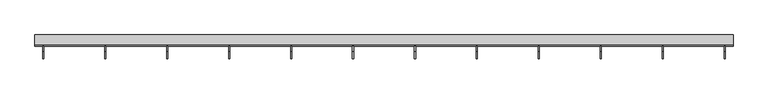
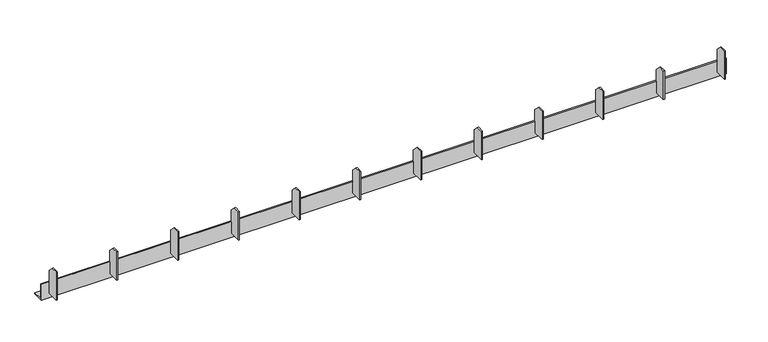
"""IFC4 building model written with IfcOpenShell, lengths in millimetres: beam geometry, NLRS_31_SF_LIB_latei geveldrager staal-AV-CWV-MMBS-SRP_gen_rsf : geveldrager_gen."""

from ifc_helpers import new_model, si_unit, frame, origin, place, context, project, spatial, polyline, outline, extrude, source, transform, mapped, element, save


def beam_0e76cdc8(model_context):
    return source(origin(), model_context, "Body", "SweptSolid", [
        extrude(outline(polyline([(-70.0, -35.0), (-180.0, -35.0), (-180.0, 235.0), (-120.0, 235.0), (-70.0, 185.0), (-70.0, -35.0)])), frame((2461.8181818, 0.0, 0.0), z_axis=(1.0, 0.0, 0.0), x_axis=(0.0, 1.0, 0.0)), (0.0, 0.0, 1.0), 10.0),
        extrude(outline(polyline([(-70.0, -35.0), (-180.0, -35.0), (-180.0, 235.0), (-120.0, 235.0), (-70.0, 185.0), (-70.0, -35.0)])), frame((1913.6363636, 0.0, 0.0), z_axis=(1.0, 0.0, 0.0), x_axis=(0.0, 1.0, 0.0)), (0.0, 0.0, 1.0), 10.0),
        extrude(outline(polyline([(-70.0, -35.0), (-180.0, -35.0), (-180.0, 235.0), (-120.0, 235.0), (-70.0, 185.0), (-70.0, -35.0)])), frame((1365.4545455, 0.0, 0.0), z_axis=(1.0, 0.0, 0.0), x_axis=(0.0, 1.0, 0.0)), (0.0, 0.0, 1.0), 10.0),
        extrude(outline(polyline([(-70.0, -35.0), (-180.0, -35.0), (-180.0, 235.0), (-120.0, 235.0), (-70.0, 185.0), (-70.0, -35.0)])), frame((817.2727273, 0.0, 0.0), z_axis=(1.0, 0.0, 0.0), x_axis=(0.0, 1.0, 0.0)), (0.0, 0.0, 1.0), 10.0),
        extrude(outline(polyline([(-70.0, -35.0), (-180.0, -35.0), (-180.0, 235.0), (-120.0, 235.0), (-70.0, 185.0), (-70.0, -35.0)])), frame((269.0909091, 0.0, 0.0), z_axis=(1.0, 0.0, 0.0), x_axis=(0.0, 1.0, 0.0)), (0.0, 0.0, 1.0), 10.0),
        extrude(outline(polyline([(-70.0, -35.0), (-180.0, -35.0), (-180.0, 235.0), (-120.0, 235.0), (-70.0, 185.0), (-70.0, -35.0)])), frame((-279.0909091, 0.0, 0.0), z_axis=(1.0, 0.0, 0.0), x_axis=(0.0, 1.0, 0.0)), (0.0, 0.0, 1.0), 10.0),
        extrude(outline(polyline([(-70.0, -35.0), (-180.0, -35.0), (-180.0, 235.0), (-120.0, 235.0), (-70.0, 185.0), (-70.0, -35.0)])), frame((-827.2727273, 0.0, 0.0), z_axis=(1.0, 0.0, 0.0), x_axis=(0.0, 1.0, 0.0)), (0.0, 0.0, 1.0), 10.0),
        extrude(outline(polyline([(-70.0, -35.0), (-180.0, -35.0), (-180.0, 235.0), (-120.0, 235.0), (-70.0, 185.0), (-70.0, -35.0)])), frame((-1375.4545455, 0.0, 0.0), z_axis=(1.0, 0.0, 0.0), x_axis=(0.0, 1.0, 0.0)), (0.0, 0.0, 1.0), 10.0),
        extrude(outline(polyline([(-70.0, -35.0), (-180.0, -35.0), (-180.0, 235.0), (-120.0, 235.0), (-70.0, 185.0), (-70.0, -35.0)])), frame((-1923.6363636, 0.0, 0.0), z_axis=(1.0, 0.0, 0.0), x_axis=(0.0, 1.0, 0.0)), (0.0, 0.0, 1.0), 10.0),
        extrude(outline(polyline([(-70.0, -35.0), (-180.0, -35.0), (-180.0, 235.0), (-120.0, 235.0), (-70.0, 185.0), (-70.0, -35.0)])), frame((-2471.8181818, 0.0, 0.0), z_axis=(1.0, 0.0, 0.0), x_axis=(0.0, 1.0, 0.0)), (0.0, 0.0, 1.0), 10.0),
        extrude(outline(polyline([(-70.0, -35.0), (-180.0, -35.0), (-180.0, 235.0), (-120.0, 235.0), (-70.0, 185.0), (-70.0, -35.0)])), frame((3010.0, 0.0, 0.0), z_axis=(1.0, 0.0, 0.0), x_axis=(0.0, 1.0, 0.0)), (0.0, 0.0, 1.0), 10.0),
        extrude(outline(polyline([(-70.0, -35.0), (-180.0, -35.0), (-180.0, 235.0), (-120.0, 235.0), (-70.0, 185.0), (-70.0, -35.0)])), frame((-3020.0, 0.0, 0.0), z_axis=(1.0, 0.0, 0.0), x_axis=(0.0, 1.0, 0.0)), (0.0, 0.0, 1.0), 10.0),
        extrude(outline(polyline([(-70.0, -75.0), (-70.0, 75.0), (-60.0, 75.0), (-60.0, -65.0), (30.0, -65.0), (30.0, -75.0), (-70.0, -75.0)])), frame((-3090.0, 0.0, 0.0), z_axis=(1.0, 0.0, 0.0), x_axis=(0.0, 1.0, 0.0)), (0.0, 0.0, 1.0), 6180.0),
    ])


if __name__ == "__main__":
    model = new_model("IFC4")
    model_context = context("Model", 3, world=origin())
    ifc_project = project(units=[si_unit("LENGTHUNIT", "METRE", prefix="MILLI")], contexts=[model_context])
    site = spatial("IfcSite", under=ifc_project)
    building = spatial("IfcBuilding", under=site)
    placement = place(None, origin())
    beam_shape = beam_0e76cdc8(model_context)
    element("IfcBeam", 1, ObjectType="NLRS_31_SF_LIB_latei geveldrager staal-AV-CWV-MMBS-SRP_gen_rsf : geveldrager_gen", at=placement, inside=building, context=model_context, shape_type="MappedRepresentation", body=[
        mapped(beam_shape, transform((0.0, 0.0, 0.0), x_axis=(1.0, 0.0, 0.0), y_axis=(0.0, 1.0, 0.0), z_axis=(0.0, 0.0, 1.0))),
    ])
    save(model, "model.ifc")

# Revit data of these elements
# Type "NLRS_31_SF_LIB_latei geveldrager staal-AV-CWV-MMBS-SRP_gen_rsf : geveldrager_gen"
#   Export Type to IFC As = "IfcBeamType"
#   Type IfcGUID = "19kvldyMP0rwUi5k27wrdj"
#   Type Comments = "geveldrager"
#   Model = "LOD200"
#   Description = "geveldrager vlgs leverancier"
#   Assembly Code = "31.10"
#   spouw_diepte [instance default] = 140 mm
#   hart_metselwerk [instance default] = 190 mm
#   r = 13 mm
#   console_hoogte [instance default] = 270 mm
#   console_eindafstand [instance default] = 75 mm
#   console_breedte [instance default] = 110 mm
#   console_beginafstand [instance default] = 75 mm
#   onderzijde_metselwerk_vanaf_vloer [instance default] = 300 mm
#   consoles_hoh [instance default] = 1000 mm
#   NLRS_C_lengte [instance default] = 1500 mm
#   Length [instance default] = 1500 mm
#   b = 100 mm
#   h = 150 mm
#   t = 10 mm
#   x = 70 mm
#   y = 75 mm
#   aantal [instance default] = 2
#   LOD300 = no
#   LOD200 = yes
#   Structural Material = NLRS_h2_staal_gen_rsf
# Element 1 (IfcBeam, "NLRS_31_SF_LIB_latei geveldrager staal-AV-CWV-MMBS-SRP_gen_rsf : geveldrager_gen")
#   consoles_hoh = 500 mm
#   NLRS_C_lengte = 6200 mm
#   aantal = 12
#   Materials on its faces: "NLRS_h2_staal_gen_rsf"
# Materials
#   "NLRS_h2_staal_gen_rsf": class "H - Metaal", colour RGB 189 187 185, transparency 0, Keynote = "h2", Manufacturer = "Revit Standards Foundation", URL = "www.revitstandards.org", Description = "staal", Cost = 0
